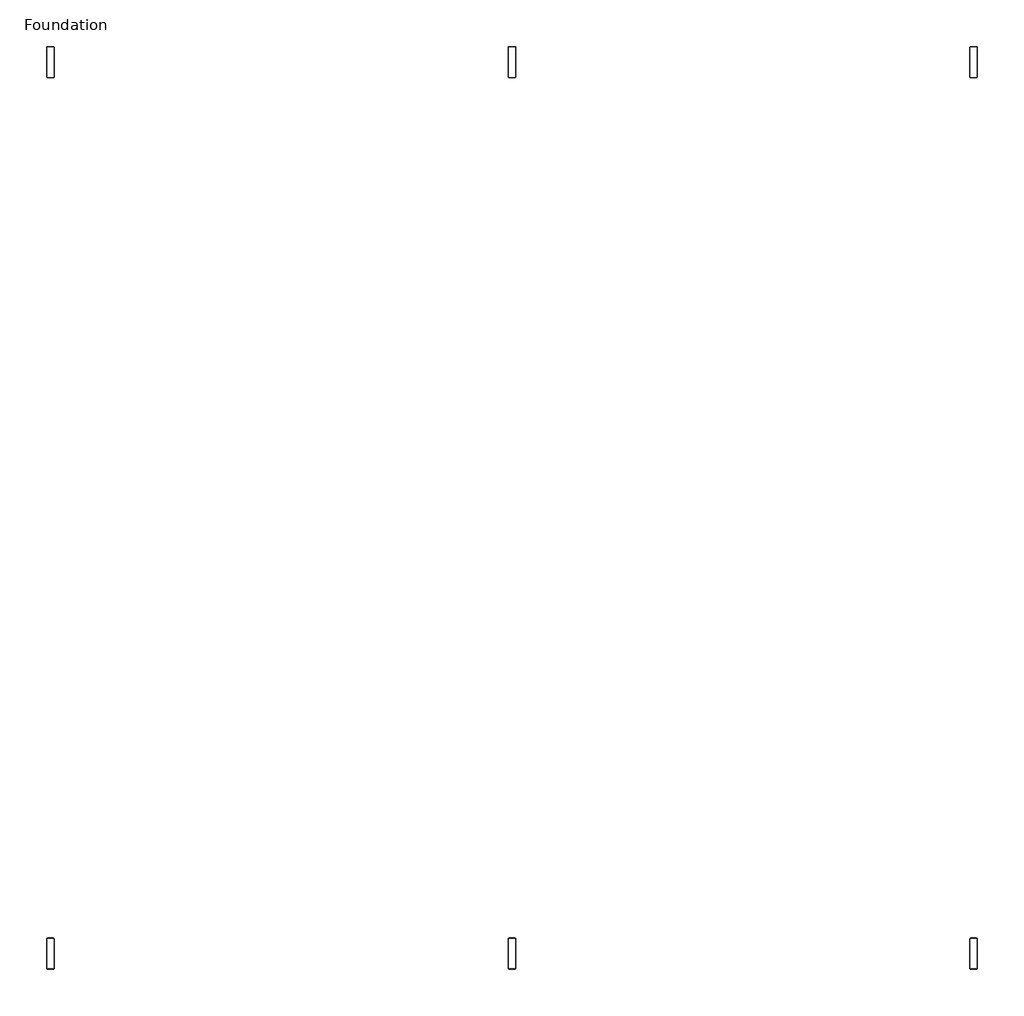
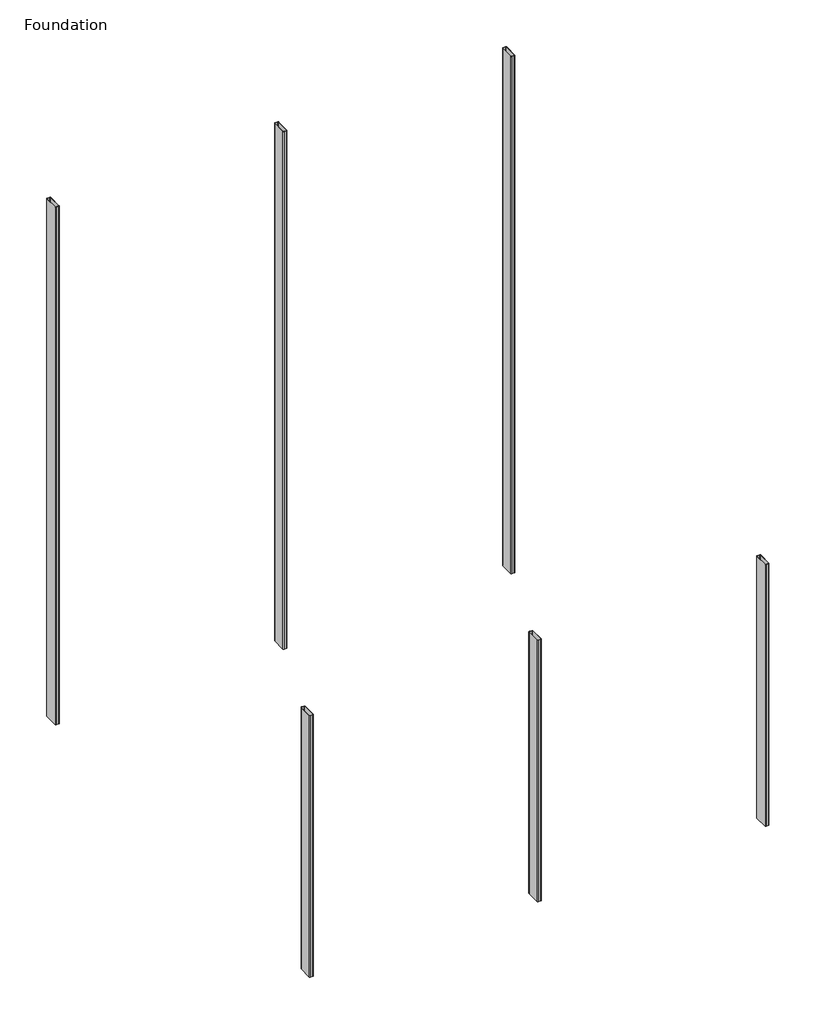
# One storey: 6 columns.
"""IFC4 building model written with IfcOpenShell, lengths in millimetres."""

import ifcopenshell
import ifcopenshell.guid

model = None  # the IFC model being written
_history = None  # IfcOwnerHistory: only IFC2X3 demands one
_inside = {}  # id of a spatial element -> (the spatial element, [elements in it])
_under = {}  # id of a project, library or spatial element -> (it, [spatial elements below it])
_declared = {}  # id of a project -> (the project, [libraries it declares])
_typed = {}  # id of a type object -> (the type object, [elements of that type])
_made_of = {}  # id of a material, layer set ... -> (it, [elements and type objects made of it])


def new_model(schema):
    """Start an empty IFC model of exactly this schema.

    Asked for "IFC4X3", IfcOpenShell would pick the latest addendum, in which some entities
    have other attributes; the version numbers below select the first issue.
    IFC2X3 requires an IfcOwnerHistory on every rooted entity: one is made here for all.
    """
    global model, _history
    if schema == "IFC4X3":
        model = ifcopenshell.file(schema_version=(4, 3, 0, 0))
    else:
        model = ifcopenshell.file(schema=schema)
    _inside.clear()
    _under.clear()
    _declared.clear()
    _typed.clear()
    _made_of.clear()
    _history = None
    if model.schema == "IFC2X3":
        org = make("IfcOrganization", Name="unknown")
        user = make(
            "IfcPersonAndOrganization",
            ThePerson=make("IfcPerson", FamilyName="unknown"),
            TheOrganization=org,
        )
        app = make(
            "IfcApplication",
            ApplicationDeveloper=org,
            Version="unknown",
            ApplicationFullName="unknown",
            ApplicationIdentifier="unknown",
        )
        _history = make(
            "IfcOwnerHistory",
            OwningUser=user,
            OwningApplication=app,
            ChangeAction="ADDED",
            CreationDate=0,
        )
    return model


def make(cls, **values):
    """One entity of the class cls with the attributes given. An attribute that is None is left unset."""
    return model.create_entity(
        cls, **{name: value for name, value in values.items() if value is not None}
    )


def rooted(cls, **values):
    """An entity with a GlobalId (a new one), such as an element, a storey or a relation."""
    return make(cls, GlobalId=ifcopenshell.guid.new(), OwnerHistory=_history, **values)


def si_unit(unit_type, name, prefix=None):
    """IfcSIUnit, for example si_unit("LENGTHUNIT", "METRE", prefix="MILLI")."""
    return make("IfcSIUnit", UnitType=unit_type, Prefix=prefix, Name=name)


def assignment(units):
    """IfcUnitAssignment: the units of a project."""
    return None if units is None else make("IfcUnitAssignment", Units=units)


def point(xyz):
    """IfcCartesianPoint."""
    return None if xyz is None else make("IfcCartesianPoint", Coordinates=xyz)


def direction(xyz):
    """IfcDirection."""
    return None if xyz is None else make("IfcDirection", DirectionRatios=xyz)


def frame(location, z_axis=None, x_axis=None):
    """IfcAxis2Placement3D, a coordinate frame: its origin and axes. An axis left out is left unset."""
    return make(
        "IfcAxis2Placement3D",
        Location=point(location),
        Axis=direction(z_axis),
        RefDirection=direction(x_axis),
    )


def frame_2d(location, x_axis=None):
    """IfcAxis2Placement2D, a coordinate frame in the plane: its origin and x axis."""
    return make(
        "IfcAxis2Placement2D", Location=point(location), RefDirection=direction(x_axis)
    )


def origin():
    """The frame at (0, 0, 0) with its axes left unset."""
    return frame((0.0, 0.0, 0.0))


def place(relative_to, where):
    """IfcLocalPlacement: puts the frame where relative to a parent placement (None: the world)."""
    return make(
        "IfcLocalPlacement", PlacementRelTo=relative_to, RelativePlacement=where
    )


def context(
    kind, dimensions, precision=None, world=None, true_north=None, identifier=None
):
    """IfcGeometricRepresentationContext, for example the 3D "Model" context."""
    return make(
        "IfcGeometricRepresentationContext",
        ContextIdentifier=identifier,
        ContextType=kind,
        CoordinateSpaceDimension=dimensions,
        Precision=precision,
        WorldCoordinateSystem=world,
        TrueNorth=true_north,
    )


def project(units=None, contexts=None):
    """IfcProject with its units and contexts."""
    return rooted(
        "IfcProject",
        Name="project",
        RepresentationContexts=contexts,
        UnitsInContext=assignment(units),
    )


def spatial(cls, under=None, at=None, **own):
    """A site, building, storey or space (cls), placed at a placement, below another one or the project."""
    s = rooted(cls, ObjectPlacement=at, **own)
    if under is not None:
        _under.setdefault(under.id(), (under, []))[1].append(s)
    return s


def polyline(points):
    """IfcPolyline through the points."""
    return make("IfcPolyline", Points=[point(p) for p in points])


def circle_curve(where, radius):
    """IfcCircle in the frame where."""
    return make("IfcCircle", Position=where, Radius=radius)


def trimmed(basis, trim1, trim2, sense, master):
    """IfcTrimmedCurve: the piece of a basis curve between two trims."""
    return make(
        "IfcTrimmedCurve",
        BasisCurve=basis,
        Trim1=trim1,
        Trim2=trim2,
        SenseAgreement=sense,
        MasterRepresentation=master,
    )


def segment(curve, same_sense, transition):
    """IfcCompositeCurveSegment."""
    return make(
        "IfcCompositeCurveSegment",
        Transition=transition,
        SameSense=same_sense,
        ParentCurve=curve,
    )


def composite_curve(segments, self_intersect=None):
    """IfcCompositeCurve: segments joined end to end."""
    return make("IfcCompositeCurve", Segments=segments, SelfIntersect=self_intersect)


def outline(outer, holes=None, kind="AREA"):
    """IfcArbitraryClosedProfileDef: a profile drawn as a closed curve; with holes, ...WithVoids."""
    if holes is None:
        return make("IfcArbitraryClosedProfileDef", ProfileType=kind, OuterCurve=outer)
    return make(
        "IfcArbitraryProfileDefWithVoids",
        ProfileType=kind,
        OuterCurve=outer,
        InnerCurves=holes,
    )


def extrude(swept, where, along, depth):
    """IfcExtrudedAreaSolid: the profile swept, set in the frame where, extruded along a direction by depth."""
    return make(
        "IfcExtrudedAreaSolid",
        SweptArea=swept,
        Position=where,
        ExtrudedDirection=direction(along),
        Depth=depth,
    )


def shape(context_of_items, identifier, shape_type, items):
    """IfcShapeRepresentation: the items that make up one representation, for example the "Body"."""
    return make(
        "IfcShapeRepresentation",
        ContextOfItems=context_of_items,
        RepresentationIdentifier=identifier,
        RepresentationType=shape_type,
        Items=items,
    )


def source(mapping_origin, context_of_items, identifier, shape_type, items):
    """IfcRepresentationMap: a shape defined once, which mapped items show again and again."""
    return make(
        "IfcRepresentationMap",
        MappingOrigin=mapping_origin,
        MappedRepresentation=shape(context_of_items, identifier, shape_type, items),
    )


def transform(
    local_origin,
    x_axis=None,
    y_axis=None,
    z_axis=None,
    scale=None,
    scale2=None,
    scale3=None,
    uniform=True,
):
    """IfcCartesianTransformationOperator3D, or its non-uniform kind. x_axis, y_axis, z_axis: its Axis1, 2, 3."""
    if uniform:
        return make(
            "IfcCartesianTransformationOperator3D",
            Axis1=direction(x_axis),
            Axis2=direction(y_axis),
            LocalOrigin=point(local_origin),
            Scale=scale,
            Axis3=direction(z_axis),
        )
    return make(
        "IfcCartesianTransformationOperator3DnonUniform",
        Axis1=direction(x_axis),
        Axis2=direction(y_axis),
        LocalOrigin=point(local_origin),
        Scale=scale,
        Axis3=direction(z_axis),
        Scale2=scale2,
        Scale3=scale3,
    )


def mapped(mapping_source, mapping_target):
    """IfcMappedItem: shows the shape of a source again, moved by a transform."""
    return make(
        "IfcMappedItem", MappingSource=mapping_source, MappingTarget=mapping_target
    )


def made_of(thing, what):
    """Note that an element or type object is made of a material, layer set ...; save() writes the relation."""
    if what is not None:
        _made_of.setdefault(what.id(), (what, []))[1].append(thing)
    return thing


def element(
    cls,
    number,
    at=None,
    inside=None,
    cuts=None,
    type_object=None,
    material=None,
    context=None,
    identifier="Body",
    shape_type=None,
    held_by="IfcProductDefinitionShape",
    body=None,
    shapes=None,
    **own,
):
    """One element of the class cls, such as IfcWall. Its Tag is "e" and its number.

    at: its placement. inside: the storey or other place that contains it. cuts: it is an
    opening in that element (IfcRelVoidsElement). A single representation is given by context,
    identifier, shape_type and body (its items); several are given by shapes. held_by: the class
    of the entity that holds the representations. save() writes the other relations.
    """
    e = rooted(cls, Tag="e%d" % number, ObjectPlacement=at, **own)
    if body is not None:
        shapes = [shape(context, identifier, shape_type, body)]
    if shapes is not None:
        e.Representation = make(held_by, Representations=shapes)
    if inside is not None:
        _inside.setdefault(inside.id(), (inside, []))[1].append(e)
    if cuts is not None:
        rooted(
            "IfcRelVoidsElement", RelatingBuildingElement=cuts, RelatedOpeningElement=e
        )
    if type_object is not None:
        _typed.setdefault(type_object.id(), (type_object, []))[1].append(e)
    return made_of(e, material)


def aggregate(whole, parts):
    """IfcRelAggregates: a whole, such as a stair, and the parts it consists of."""
    return rooted("IfcRelAggregates", RelatingObject=whole, RelatedObjects=parts)


def save(model, path):
    """Write the relations noted so far, then the file.

    IfcRelAggregates (storeys below a building ...), IfcRelContainedInSpatialStructure (elements
    in a storey), IfcRelDefinesByType, IfcRelAssociatesMaterial and IfcRelDeclares: one each for
    every whole, place, type object, material and project.
    """
    for whole, parts in _under.values():
        aggregate(whole, parts)
    for where, things in _inside.values():
        rooted(
            "IfcRelContainedInSpatialStructure",
            RelatedElements=things,
            RelatingStructure=where,
        )
    for kind, things in _typed.values():
        rooted("IfcRelDefinesByType", RelatedObjects=things, RelatingType=kind)
    for what, things in _made_of.values():
        rooted("IfcRelAssociatesMaterial", RelatedObjects=things, RelatingMaterial=what)
    for by, libraries in _declared.values():
        rooted("IfcRelDeclares", RelatingContext=by, RelatedDefinitions=libraries)
    model.write(path)


def hss_hollow_structural_section_column_hss8x2x3_16_e881e9b5(model_context):
    return source(origin(), model_context, "Body", "SweptSolid", [
        extrude(outline(composite_curve([segment(trimmed(circle_curve(frame_2d((16.5608, 92.7608)), 8.8392), [point((16.5608, 101.6))], [point((25.4, 92.7608))], False, "CARTESIAN"), True, "CONTINUOUS"), segment(polyline([(25.4, 92.7608), (25.4, -92.7608)]), True, "CONTINUOUS"), segment(trimmed(circle_curve(frame_2d((16.5608, -92.7608)), 8.8392), [point((25.4, -92.7608))], [point((16.5608, -101.6))], False, "CARTESIAN"), True, "CONTINUOUS"), segment(polyline([(16.5608, -101.6), (-16.5608, -101.6)]), True, "CONTINUOUS"), segment(trimmed(circle_curve(frame_2d((-16.5608, -92.7608)), 8.8392), [point((-16.5608, -101.6))], [point((-25.4, -92.7608))], False, "CARTESIAN"), True, "CONTINUOUS"), segment(polyline([(-25.4, -92.7608), (-25.4, 92.7608)]), True, "CONTINUOUS"), segment(trimmed(circle_curve(frame_2d((-16.5608, 92.7608)), 8.8392), [point((-25.4, 92.7608))], [point((-16.5608, 101.6))], False, "CARTESIAN"), True, "CONTINUOUS"), segment(polyline([(-16.5608, 101.6), (16.5608, 101.6)]), True, "CONTINUOUS")], self_intersect=False), holes=[composite_curve([segment(polyline([(16.5608, 97.1804), (-16.5608, 97.1804)]), True, "CONTINUOUS"), segment(trimmed(circle_curve(frame_2d((-16.5608, 92.7608)), 4.4196), [point((-16.5608, 97.1804))], [point((-20.9804, 92.7608))], True, "CARTESIAN"), True, "CONTINUOUS"), segment(polyline([(-20.9804, 92.7608), (-20.9804, -92.7608)]), True, "CONTINUOUS"), segment(trimmed(circle_curve(frame_2d((-16.5608, -92.7608)), 4.4196), [point((-20.9804, -92.7608))], [point((-16.5608, -97.1804))], True, "CARTESIAN"), True, "CONTINUOUS"), segment(polyline([(-16.5608, -97.1804), (16.5608, -97.1804)]), True, "CONTINUOUS"), segment(trimmed(circle_curve(frame_2d((16.5608, -92.7608)), 4.4196), [point((16.5608, -97.1804))], [point((20.9804, -92.7608))], True, "CARTESIAN"), True, "CONTINUOUS"), segment(polyline([(20.9804, -92.7608), (20.9804, 92.7608)]), True, "CONTINUOUS"), segment(trimmed(circle_curve(frame_2d((16.5608, 92.7608)), 4.4196), [point((20.9804, 92.7608))], [point((16.5608, 97.1804))], True, "CARTESIAN"), True, "CONTINUOUS")], self_intersect=False)]), frame((0.0, 0.0, -1200.0), z_axis=(0.0, 0.0, 1.0), x_axis=(1.0, 0.0, 0.0)), (0.0, 0.0, 1.0), 7200.0),
    ])


def hss_hollow_structural_section_column_hss8x2x3_16_13fa7c93(model_context):
    return source(origin(), model_context, "Body", "SweptSolid", [
        extrude(outline(composite_curve([segment(trimmed(circle_curve(frame_2d((16.5608, 92.7608)), 8.8392), [point((16.5608, 101.6))], [point((25.4, 92.7608))], False, "CARTESIAN"), True, "CONTINUOUS"), segment(polyline([(25.4, 92.7608), (25.4, -92.7608)]), True, "CONTINUOUS"), segment(trimmed(circle_curve(frame_2d((16.5608, -92.7608)), 8.8392), [point((25.4, -92.7608))], [point((16.5608, -101.6))], False, "CARTESIAN"), True, "CONTINUOUS"), segment(polyline([(16.5608, -101.6), (-16.5608, -101.6)]), True, "CONTINUOUS"), segment(trimmed(circle_curve(frame_2d((-16.5608, -92.7608)), 8.8392), [point((-16.5608, -101.6))], [point((-25.4, -92.7608))], False, "CARTESIAN"), True, "CONTINUOUS"), segment(polyline([(-25.4, -92.7608), (-25.4, 92.7608)]), True, "CONTINUOUS"), segment(trimmed(circle_curve(frame_2d((-16.5608, 92.7608)), 8.8392), [point((-25.4, 92.7608))], [point((-16.5608, 101.6))], False, "CARTESIAN"), True, "CONTINUOUS"), segment(polyline([(-16.5608, 101.6), (16.5608, 101.6)]), True, "CONTINUOUS")], self_intersect=False), holes=[composite_curve([segment(polyline([(16.5608, 97.1804), (-16.5608, 97.1804)]), True, "CONTINUOUS"), segment(trimmed(circle_curve(frame_2d((-16.5608, 92.7608)), 4.4196), [point((-16.5608, 97.1804))], [point((-20.9804, 92.7608))], True, "CARTESIAN"), True, "CONTINUOUS"), segment(polyline([(-20.9804, 92.7608), (-20.9804, -92.7608)]), True, "CONTINUOUS"), segment(trimmed(circle_curve(frame_2d((-16.5608, -92.7608)), 4.4196), [point((-20.9804, -92.7608))], [point((-16.5608, -97.1804))], True, "CARTESIAN"), True, "CONTINUOUS"), segment(polyline([(-16.5608, -97.1804), (16.5608, -97.1804)]), True, "CONTINUOUS"), segment(trimmed(circle_curve(frame_2d((16.5608, -92.7608)), 4.4196), [point((16.5608, -97.1804))], [point((20.9804, -92.7608))], True, "CARTESIAN"), True, "CONTINUOUS"), segment(polyline([(20.9804, -92.7608), (20.9804, 92.7608)]), True, "CONTINUOUS"), segment(trimmed(circle_curve(frame_2d((16.5608, 92.7608)), 4.4196), [point((20.9804, 92.7608))], [point((16.5608, 97.1804))], True, "CARTESIAN"), True, "CONTINUOUS")], self_intersect=False)]), frame((0.0, 0.0, -1200.0), z_axis=(0.0, 0.0, 1.0), x_axis=(1.0, 0.0, 0.0)), (0.0, 0.0, 1.0), 3639.0),
    ])


def hss_hollow_structural_section_column_hss8x2x3_16_47370f60(model_context):
    return source(origin(), model_context, "Body", "SweptSolid", [
        extrude(outline(composite_curve([segment(trimmed(circle_curve(frame_2d((16.5608, 92.7608)), 8.8392), [point((16.5608, 101.6))], [point((25.4, 92.7608))], False, "CARTESIAN"), True, "CONTINUOUS"), segment(polyline([(25.4, 92.7608), (25.4, -92.7608)]), True, "CONTINUOUS"), segment(trimmed(circle_curve(frame_2d((16.5608, -92.7608)), 8.8392), [point((25.4, -92.7608))], [point((16.5608, -101.6))], False, "CARTESIAN"), True, "CONTINUOUS"), segment(polyline([(16.5608, -101.6), (-16.5608, -101.6)]), True, "CONTINUOUS"), segment(trimmed(circle_curve(frame_2d((-16.5608, -92.7608)), 8.8392), [point((-16.5608, -101.6))], [point((-25.4, -92.7608))], False, "CARTESIAN"), True, "CONTINUOUS"), segment(polyline([(-25.4, -92.7608), (-25.4, 92.7608)]), True, "CONTINUOUS"), segment(trimmed(circle_curve(frame_2d((-16.5608, 92.7608)), 8.8392), [point((-25.4, 92.7608))], [point((-16.5608, 101.6))], False, "CARTESIAN"), True, "CONTINUOUS"), segment(polyline([(-16.5608, 101.6), (16.5608, 101.6)]), True, "CONTINUOUS")], self_intersect=False), holes=[composite_curve([segment(polyline([(16.5608, 97.1804), (-16.5608, 97.1804)]), True, "CONTINUOUS"), segment(trimmed(circle_curve(frame_2d((-16.5608, 92.7608)), 4.4196), [point((-16.5608, 97.1804))], [point((-20.9804, 92.7608))], True, "CARTESIAN"), True, "CONTINUOUS"), segment(polyline([(-20.9804, 92.7608), (-20.9804, -92.7608)]), True, "CONTINUOUS"), segment(trimmed(circle_curve(frame_2d((-16.5608, -92.7608)), 4.4196), [point((-20.9804, -92.7608))], [point((-16.5608, -97.1804))], True, "CARTESIAN"), True, "CONTINUOUS"), segment(polyline([(-16.5608, -97.1804), (16.5608, -97.1804)]), True, "CONTINUOUS"), segment(trimmed(circle_curve(frame_2d((16.5608, -92.7608)), 4.4196), [point((16.5608, -97.1804))], [point((20.9804, -92.7608))], True, "CARTESIAN"), True, "CONTINUOUS"), segment(polyline([(20.9804, -92.7608), (20.9804, 92.7608)]), True, "CONTINUOUS"), segment(trimmed(circle_curve(frame_2d((16.5608, 92.7608)), 4.4196), [point((20.9804, 92.7608))], [point((16.5608, 97.1804))], True, "CARTESIAN"), True, "CONTINUOUS")], self_intersect=False)]), frame((0.0, 0.0, -1200.0), z_axis=(0.0, 0.0, 1.0), x_axis=(1.0, 0.0, 0.0)), (0.0, 0.0, 1.0), 3644.0),
    ])


def hss_hollow_structural_section_column_hss8x2x3_16_3803074a(model_context):
    return source(origin(), model_context, "Body", "SweptSolid", [
        extrude(outline(composite_curve([segment(trimmed(circle_curve(frame_2d((16.5608, 92.7608)), 8.8392), [point((16.5608, 101.6))], [point((25.4, 92.7608))], False, "CARTESIAN"), True, "CONTINUOUS"), segment(polyline([(25.4, 92.7608), (25.4, -92.7608)]), True, "CONTINUOUS"), segment(trimmed(circle_curve(frame_2d((16.5608, -92.7608)), 8.8392), [point((25.4, -92.7608))], [point((16.5608, -101.6))], False, "CARTESIAN"), True, "CONTINUOUS"), segment(polyline([(16.5608, -101.6), (-16.5608, -101.6)]), True, "CONTINUOUS"), segment(trimmed(circle_curve(frame_2d((-16.5608, -92.7608)), 8.8392), [point((-16.5608, -101.6))], [point((-25.4, -92.7608))], False, "CARTESIAN"), True, "CONTINUOUS"), segment(polyline([(-25.4, -92.7608), (-25.4, 92.7608)]), True, "CONTINUOUS"), segment(trimmed(circle_curve(frame_2d((-16.5608, 92.7608)), 8.8392), [point((-25.4, 92.7608))], [point((-16.5608, 101.6))], False, "CARTESIAN"), True, "CONTINUOUS"), segment(polyline([(-16.5608, 101.6), (16.5608, 101.6)]), True, "CONTINUOUS")], self_intersect=False), holes=[composite_curve([segment(polyline([(16.5608, 97.1804), (-16.5608, 97.1804)]), True, "CONTINUOUS"), segment(trimmed(circle_curve(frame_2d((-16.5608, 92.7608)), 4.4196), [point((-16.5608, 97.1804))], [point((-20.9804, 92.7608))], True, "CARTESIAN"), True, "CONTINUOUS"), segment(polyline([(-20.9804, 92.7608), (-20.9804, -92.7608)]), True, "CONTINUOUS"), segment(trimmed(circle_curve(frame_2d((-16.5608, -92.7608)), 4.4196), [point((-20.9804, -92.7608))], [point((-16.5608, -97.1804))], True, "CARTESIAN"), True, "CONTINUOUS"), segment(polyline([(-16.5608, -97.1804), (16.5608, -97.1804)]), True, "CONTINUOUS"), segment(trimmed(circle_curve(frame_2d((16.5608, -92.7608)), 4.4196), [point((16.5608, -97.1804))], [point((20.9804, -92.7608))], True, "CARTESIAN"), True, "CONTINUOUS"), segment(polyline([(20.9804, -92.7608), (20.9804, 92.7608)]), True, "CONTINUOUS"), segment(trimmed(circle_curve(frame_2d((16.5608, 92.7608)), 4.4196), [point((20.9804, 92.7608))], [point((16.5608, 97.1804))], True, "CARTESIAN"), True, "CONTINUOUS")], self_intersect=False)]), frame((0.0, 0.0, -1200.0), z_axis=(0.0, 0.0, 1.0), x_axis=(1.0, 0.0, 0.0)), (0.0, 0.0, 1.0), 7205.0),
    ])


model = new_model("IFC4")

# Units and contexts
model_context = context("Model", 3, world=origin())
ifc_project = project(units=[si_unit("LENGTHUNIT", "METRE", prefix="MILLI")], contexts=[model_context])

# Site, building, storey
site = spatial("IfcSite", under=ifc_project)
building = spatial("IfcBuilding", under=site)
storey = spatial("IfcBuildingStorey", under=building, Name="Foundation", Elevation=-1200.0)

# Columns
placement = place(None, origin())
hss_hollow_structural_section_column_hss8x2x3_16_shape = hss_hollow_structural_section_column_hss8x2x3_16_e881e9b5(model_context)
element("IfcColumn", 1, ObjectType="HSS-Hollow Structural Section-Column : HSS8X2X3/16", at=placement, inside=storey, context=model_context, shape_type="MappedRepresentation", body=[
    mapped(hss_hollow_structural_section_column_hss8x2x3_16_shape, transform((13061.9315174, 2696.9060214, 0.0), x_axis=(-1.0, 0.0, 0.0), y_axis=(0.0, -1.0, 0.0), z_axis=(0.0, 0.0, 1.0))),
])
hss_hollow_structural_section_column_hss8x2x3_16_2_shape = hss_hollow_structural_section_column_hss8x2x3_16_13fa7c93(model_context)
element("IfcColumn", 2, ObjectType="HSS-Hollow Structural Section-Column : HSS8X2X3/16", at=placement, inside=storey, context=model_context, shape_type="MappedRepresentation", body=[
    mapped(hss_hollow_structural_section_column_hss8x2x3_16_2_shape, transform((10061.9315174, -3100.0939786, 0.0), x_axis=(-1.0, 0.0, 0.0), y_axis=(0.0, -1.0, 0.0), z_axis=(0.0, 0.0, 1.0))),
])
element("IfcColumn", 3, ObjectType="HSS-Hollow Structural Section-Column : HSS8X2X3/16", at=placement, inside=storey, context=model_context, shape_type="MappedRepresentation", body=[
    mapped(hss_hollow_structural_section_column_hss8x2x3_16_2_shape, transform((7061.9315174, -3100.0939786, 0.0), x_axis=(-1.0, 0.0, 0.0), y_axis=(0.0, -1.0, 0.0), z_axis=(0.0, 0.0, 1.0))),
])
hss_hollow_structural_section_column_hss8x2x3_16_3_shape = hss_hollow_structural_section_column_hss8x2x3_16_47370f60(model_context)
element("IfcColumn", 4, ObjectType="HSS-Hollow Structural Section-Column : HSS8X2X3/16", at=placement, inside=storey, context=model_context, shape_type="MappedRepresentation", body=[
    mapped(hss_hollow_structural_section_column_hss8x2x3_16_3_shape, transform((13061.9315174, -3100.0939786, 0.0), x_axis=(-1.0, 0.0, 0.0), y_axis=(0.0, -1.0, 0.0), z_axis=(0.0, 0.0, 1.0))),
])
hss_hollow_structural_section_column_hss8x2x3_16_4_shape = hss_hollow_structural_section_column_hss8x2x3_16_3803074a(model_context)
element("IfcColumn", 5, ObjectType="HSS-Hollow Structural Section-Column : HSS8X2X3/16", at=placement, inside=storey, context=model_context, shape_type="MappedRepresentation", body=[
    mapped(hss_hollow_structural_section_column_hss8x2x3_16_4_shape, transform((10061.9315174, 2696.9060214, 0.0), x_axis=(-1.0, 0.0, 0.0), y_axis=(0.0, -1.0, 0.0), z_axis=(0.0, 0.0, 1.0))),
])
element("IfcColumn", 6, ObjectType="HSS-Hollow Structural Section-Column : HSS8X2X3/16", at=placement, inside=storey, context=model_context, shape_type="MappedRepresentation", body=[
    mapped(hss_hollow_structural_section_column_hss8x2x3_16_4_shape, transform((7061.9315174, 2696.9060214, 0.0), x_axis=(-1.0, 0.0, 0.0), y_axis=(0.0, -1.0, 0.0), z_axis=(0.0, 0.0, 1.0))),
])

save(model, "model.ifc")

# Revit data of these elements
# Project information
#   Project Issue Date = "Issue Date"
#   Project Status = "Project Status"
#   Client Name = "Owner"
#   Project Address = "Enter address here"
#   Project Name = "Project Name"
#   Project Number = "0001"
# Type "HSS-Hollow Structural Section-Column : HSS8X2X3/16"
#   Assembly Code = "B10"
#   Shape = "Rect."
#   Cost = 1
#   W = 12
#   Ht = 203.2 mm
#   b = 50.8 mm
#   kr = 8.839 mm
#   t = 4.42 mm
#   A = 0.00211612 m²
#   Structural Material [instance default] = Steel ASTM A500, Grade B, Rectangular and Square
# Elements 1, 2, 3, 4, 5, 6 (IfcColumn, "HSS-Hollow Structural Section-Column : HSS8X2X3/16")
#   Structural Material = Metal - Steel 43-275
#   Phase Created = New Construction
#   Materials on its faces: "Metal - Steel 43-275"
# Materials
#   "Steel ASTM A500, Grade B, Rectangular and Square": class "Metal", colour RGB 199 199 199, transparency 0, Description = "Carbon steel", Cost = 0
#   "Metal - Steel 43-275": class "Metal", colour RGB 247 247 247, transparency 0, Cost = 0
